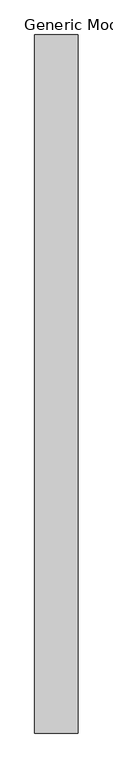
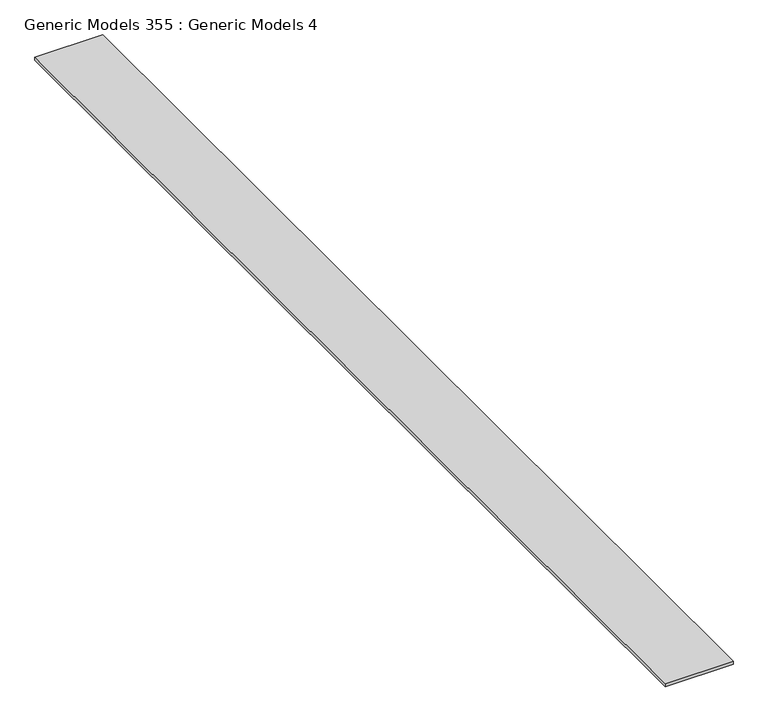
"""IFC4 building model written with IfcOpenShell, lengths in millimetres: proxy geometry, Generic Models 355 : Generic Models 4."""

import ifcopenshell
import ifcopenshell.guid

model = None  # the IFC model being written
_history = None  # IfcOwnerHistory: only IFC2X3 demands one
_inside = {}  # id of a spatial element -> (the spatial element, [elements in it])
_under = {}  # id of a project, library or spatial element -> (it, [spatial elements below it])
_declared = {}  # id of a project -> (the project, [libraries it declares])
_typed = {}  # id of a type object -> (the type object, [elements of that type])
_made_of = {}  # id of a material, layer set ... -> (it, [elements and type objects made of it])


def new_model(schema):
    """Start an empty IFC model of exactly this schema.

    Asked for "IFC4X3", IfcOpenShell would pick the latest addendum, in which some entities
    have other attributes; the version numbers below select the first issue.
    IFC2X3 requires an IfcOwnerHistory on every rooted entity: one is made here for all.
    """
    global model, _history
    if schema == "IFC4X3":
        model = ifcopenshell.file(schema_version=(4, 3, 0, 0))
    else:
        model = ifcopenshell.file(schema=schema)
    _inside.clear()
    _under.clear()
    _declared.clear()
    _typed.clear()
    _made_of.clear()
    _history = None
    if model.schema == "IFC2X3":
        org = make("IfcOrganization", Name="unknown")
        user = make(
            "IfcPersonAndOrganization",
            ThePerson=make("IfcPerson", FamilyName="unknown"),
            TheOrganization=org,
        )
        app = make(
            "IfcApplication",
            ApplicationDeveloper=org,
            Version="unknown",
            ApplicationFullName="unknown",
            ApplicationIdentifier="unknown",
        )
        _history = make(
            "IfcOwnerHistory",
            OwningUser=user,
            OwningApplication=app,
            ChangeAction="ADDED",
            CreationDate=0,
        )
    return model


def make(cls, **values):
    """One entity of the class cls with the attributes given. An attribute that is None is left unset."""
    return model.create_entity(
        cls, **{name: value for name, value in values.items() if value is not None}
    )


def rooted(cls, **values):
    """An entity with a GlobalId (a new one), such as an element, a storey or a relation."""
    return make(cls, GlobalId=ifcopenshell.guid.new(), OwnerHistory=_history, **values)


def si_unit(unit_type, name, prefix=None):
    """IfcSIUnit, for example si_unit("LENGTHUNIT", "METRE", prefix="MILLI")."""
    return make("IfcSIUnit", UnitType=unit_type, Prefix=prefix, Name=name)


def assignment(units):
    """IfcUnitAssignment: the units of a project."""
    return None if units is None else make("IfcUnitAssignment", Units=units)


def point(xyz):
    """IfcCartesianPoint."""
    return None if xyz is None else make("IfcCartesianPoint", Coordinates=xyz)


def direction(xyz):
    """IfcDirection."""
    return None if xyz is None else make("IfcDirection", DirectionRatios=xyz)


def frame(location, z_axis=None, x_axis=None):
    """IfcAxis2Placement3D, a coordinate frame: its origin and axes. An axis left out is left unset."""
    return make(
        "IfcAxis2Placement3D",
        Location=point(location),
        Axis=direction(z_axis),
        RefDirection=direction(x_axis),
    )


def origin():
    """The frame at (0, 0, 0) with its axes left unset."""
    return frame((0.0, 0.0, 0.0))


def place(relative_to, where):
    """IfcLocalPlacement: puts the frame where relative to a parent placement (None: the world)."""
    return make(
        "IfcLocalPlacement", PlacementRelTo=relative_to, RelativePlacement=where
    )


def context(
    kind, dimensions, precision=None, world=None, true_north=None, identifier=None
):
    """IfcGeometricRepresentationContext, for example the 3D "Model" context."""
    return make(
        "IfcGeometricRepresentationContext",
        ContextIdentifier=identifier,
        ContextType=kind,
        CoordinateSpaceDimension=dimensions,
        Precision=precision,
        WorldCoordinateSystem=world,
        TrueNorth=true_north,
    )


def project(units=None, contexts=None):
    """IfcProject with its units and contexts."""
    return rooted(
        "IfcProject",
        Name="project",
        RepresentationContexts=contexts,
        UnitsInContext=assignment(units),
    )


def spatial(cls, under=None, at=None, **own):
    """A site, building, storey or space (cls), placed at a placement, below another one or the project."""
    s = rooted(cls, ObjectPlacement=at, **own)
    if under is not None:
        _under.setdefault(under.id(), (under, []))[1].append(s)
    return s


def polyline(points):
    """IfcPolyline through the points."""
    return make("IfcPolyline", Points=[point(p) for p in points])


def outline(outer, holes=None, kind="AREA"):
    """IfcArbitraryClosedProfileDef: a profile drawn as a closed curve; with holes, ...WithVoids."""
    if holes is None:
        return make("IfcArbitraryClosedProfileDef", ProfileType=kind, OuterCurve=outer)
    return make(
        "IfcArbitraryProfileDefWithVoids",
        ProfileType=kind,
        OuterCurve=outer,
        InnerCurves=holes,
    )


def extrude(swept, where, along, depth):
    """IfcExtrudedAreaSolid: the profile swept, set in the frame where, extruded along a direction by depth."""
    return make(
        "IfcExtrudedAreaSolid",
        SweptArea=swept,
        Position=where,
        ExtrudedDirection=direction(along),
        Depth=depth,
    )


def shape(context_of_items, identifier, shape_type, items):
    """IfcShapeRepresentation: the items that make up one representation, for example the "Body"."""
    return make(
        "IfcShapeRepresentation",
        ContextOfItems=context_of_items,
        RepresentationIdentifier=identifier,
        RepresentationType=shape_type,
        Items=items,
    )


def source(mapping_origin, context_of_items, identifier, shape_type, items):
    """IfcRepresentationMap: a shape defined once, which mapped items show again and again."""
    return make(
        "IfcRepresentationMap",
        MappingOrigin=mapping_origin,
        MappedRepresentation=shape(context_of_items, identifier, shape_type, items),
    )


def transform(
    local_origin,
    x_axis=None,
    y_axis=None,
    z_axis=None,
    scale=None,
    scale2=None,
    scale3=None,
    uniform=True,
):
    """IfcCartesianTransformationOperator3D, or its non-uniform kind. x_axis, y_axis, z_axis: its Axis1, 2, 3."""
    if uniform:
        return make(
            "IfcCartesianTransformationOperator3D",
            Axis1=direction(x_axis),
            Axis2=direction(y_axis),
            LocalOrigin=point(local_origin),
            Scale=scale,
            Axis3=direction(z_axis),
        )
    return make(
        "IfcCartesianTransformationOperator3DnonUniform",
        Axis1=direction(x_axis),
        Axis2=direction(y_axis),
        LocalOrigin=point(local_origin),
        Scale=scale,
        Axis3=direction(z_axis),
        Scale2=scale2,
        Scale3=scale3,
    )


def mapped(mapping_source, mapping_target):
    """IfcMappedItem: shows the shape of a source again, moved by a transform."""
    return make(
        "IfcMappedItem", MappingSource=mapping_source, MappingTarget=mapping_target
    )


def made_of(thing, what):
    """Note that an element or type object is made of a material, layer set ...; save() writes the relation."""
    if what is not None:
        _made_of.setdefault(what.id(), (what, []))[1].append(thing)
    return thing


def element(
    cls,
    number,
    at=None,
    inside=None,
    cuts=None,
    type_object=None,
    material=None,
    context=None,
    identifier="Body",
    shape_type=None,
    held_by="IfcProductDefinitionShape",
    body=None,
    shapes=None,
    **own,
):
    """One element of the class cls, such as IfcWall. Its Tag is "e" and its number.

    at: its placement. inside: the storey or other place that contains it. cuts: it is an
    opening in that element (IfcRelVoidsElement). A single representation is given by context,
    identifier, shape_type and body (its items); several are given by shapes. held_by: the class
    of the entity that holds the representations. save() writes the other relations.
    """
    e = rooted(cls, Tag="e%d" % number, ObjectPlacement=at, **own)
    if body is not None:
        shapes = [shape(context, identifier, shape_type, body)]
    if shapes is not None:
        e.Representation = make(held_by, Representations=shapes)
    if inside is not None:
        _inside.setdefault(inside.id(), (inside, []))[1].append(e)
    if cuts is not None:
        rooted(
            "IfcRelVoidsElement", RelatingBuildingElement=cuts, RelatedOpeningElement=e
        )
    if type_object is not None:
        _typed.setdefault(type_object.id(), (type_object, []))[1].append(e)
    return made_of(e, material)


def aggregate(whole, parts):
    """IfcRelAggregates: a whole, such as a stair, and the parts it consists of."""
    return rooted("IfcRelAggregates", RelatingObject=whole, RelatedObjects=parts)


def save(model, path):
    """Write the relations noted so far, then the file.

    IfcRelAggregates (storeys below a building ...), IfcRelContainedInSpatialStructure (elements
    in a storey), IfcRelDefinesByType, IfcRelAssociatesMaterial and IfcRelDeclares: one each for
    every whole, place, type object, material and project.
    """
    for whole, parts in _under.values():
        aggregate(whole, parts)
    for where, things in _inside.values():
        rooted(
            "IfcRelContainedInSpatialStructure",
            RelatedElements=things,
            RelatingStructure=where,
        )
    for kind, things in _typed.values():
        rooted("IfcRelDefinesByType", RelatedObjects=things, RelatingType=kind)
    for what, things in _made_of.values():
        rooted("IfcRelAssociatesMaterial", RelatedObjects=things, RelatingMaterial=what)
    for by, libraries in _declared.values():
        rooted("IfcRelDeclares", RelatingContext=by, RelatedDefinitions=libraries)
    model.write(path)


def generic_models_355_generic_models_4_63cbbe1a(model_context):
    return source(origin(), model_context, "Body", "SweptSolid", [
        extrude(outline(polyline([(10069.8245523, -6864.9230338), (9671.8363263, -6864.9230338), (9671.8363263, -464.1230338), (10069.8245523, -464.1230338), (10069.8245523, -6864.9230338)])), frame((0.0, 0.0, 126524.8520404), z_axis=(0.0, 0.0, 1.0), x_axis=(1.0, 0.0, 0.0)), (0.0, 0.0, 1.0), 19.05),
    ])


if __name__ == "__main__":
    model = new_model("IFC4")
    model_context = context("Model", 3, world=origin())
    ifc_project = project(units=[si_unit("LENGTHUNIT", "METRE", prefix="MILLI")], contexts=[model_context])
    site = spatial("IfcSite", under=ifc_project)
    building = spatial("IfcBuilding", under=site)
    placement = place(None, origin())
    generic_models_355_generic_models_4_shape = generic_models_355_generic_models_4_63cbbe1a(model_context)
    element("IfcBuildingElementProxy", 1, Name="Generic Models 355 : Generic Models 4", ObjectType="Generic Models 355 : Generic Models 4", at=placement, inside=building, context=model_context, shape_type="MappedRepresentation", body=[
        mapped(generic_models_355_generic_models_4_shape, transform((0.0, 0.0, 0.0), x_axis=(1.0, 0.0, 0.0), y_axis=(0.0, 1.0, 0.0), z_axis=(0.0, 0.0, 1.0))),
    ])
    save(model, "model.ifc")

# Revit data of these elements
# Element 1 (IfcBuildingElementProxy, "Generic Models 355 : Generic Models 4")
#   Materials on its faces: "_CDX PLYWOOD - SEE STRUCT DWGs"
# Materials
#   "_CDX PLYWOOD - SEE STRUCT DWGs": class "Generic", colour RGB 98 75 74, transparency 0, Cost = 0
